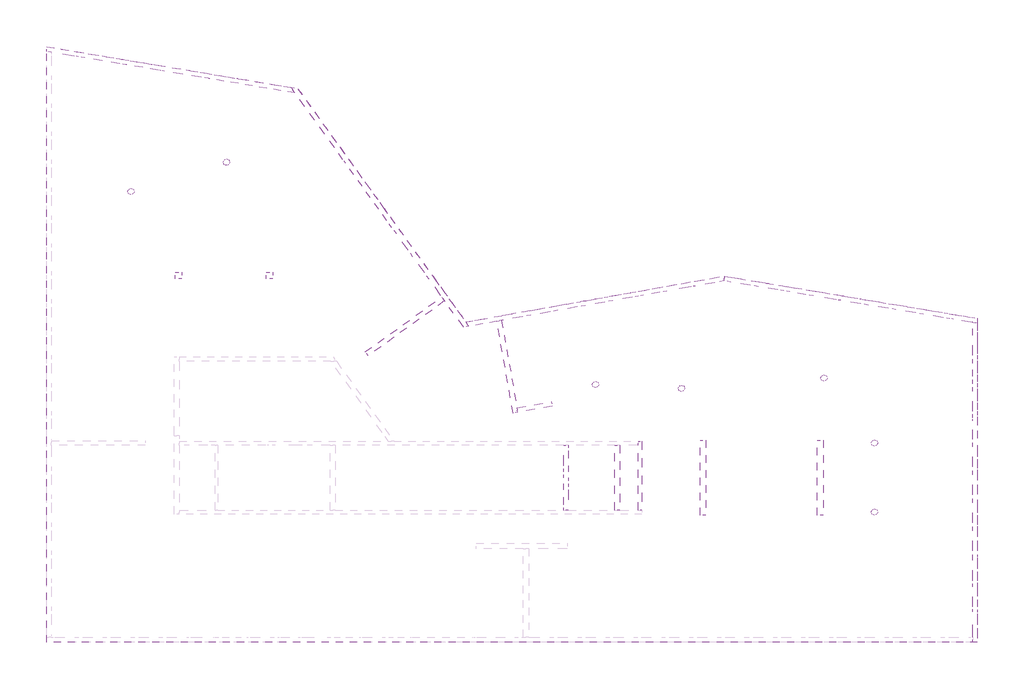
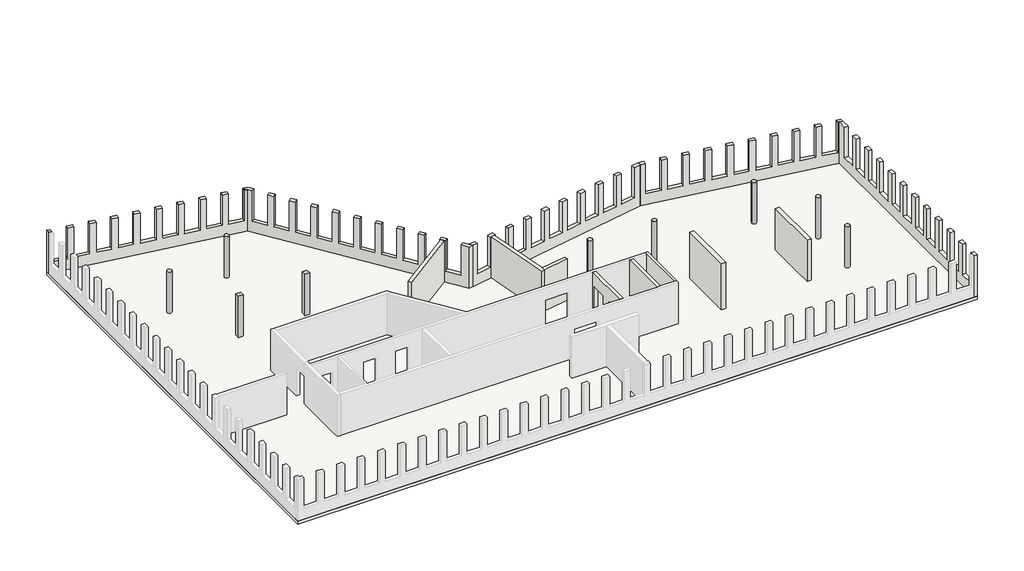
# One storey, part 2 of 2: 13 walls, 9 columns, 1 slab.
"""IFC4 building model written with IfcOpenShell, lengths in millimetres."""

from ifc_helpers import new_model, si_unit, point, frame, frame_2d, origin, place, context, project, spatial, polyline, circle_curve, trimmed, segment, composite_curve, outline, extrude, faceted_brep, element, save

model = new_model("IFC4")

# Units and contexts
model_context = context("Model", 3, world=origin())
ifc_project = project(units=[si_unit("LENGTHUNIT", "METRE", prefix="MILLI")], contexts=[model_context])

# Site, building, storey
site = spatial("IfcSite", under=ifc_project)
building = spatial("IfcBuilding", under=site)
storey = spatial("IfcBuildingStorey", under=building, Name="03_OG_OKFB_10,38", Elevation=10380.0)

# Columns
placement = place(None, origin())
element("IfcColumn", 1, ObjectType="5dki STB-Stützen rund : 5dki Stütze rund ø35cm C40/50", at=placement, inside=storey, context=model_context, shape_type="SweptSolid", body=[
    extrude(outline(composite_curve([segment(trimmed(circle_curve(frame_2d((33961.7583834, 13503.0230367)), 175.0), [point((34136.7583834, 13503.0230367))], [point((33786.7583834, 13503.0230367))], False, "CARTESIAN"), True, "CONTINUOUS"), segment(trimmed(circle_curve(frame_2d((33961.7583834, 13503.0230367)), 175.0), [point((33786.7583834, 13503.0230367))], [point((34136.7583834, 13503.0230367))], False, "CARTESIAN"), True, "CONTINUOUS")], self_intersect=False)), frame((0.0, 0.0, 13690.0), z_axis=(0.0, 0.0, 1.0), x_axis=(1.0, 0.0, 0.0)), (0.0, 0.0, 1.0), 3210.0),
])
element("IfcColumn", 2, ObjectType="5dki STB-Stützen rechteckig : 5dki Stütze recht. 35x35cm C35/45", at=placement, inside=storey, context=model_context, shape_type="SweptSolid", body=[
    extrude(outline(polyline([(7139.9999521, 19742.0124565), (7139.9999521, 19392.0124565), (6789.9999521, 19392.0124565), (6789.9999521, 19742.0124565), (7139.9999521, 19742.0124565)])), frame((0.0, 0.0, 13690.0), z_axis=(0.0, 0.0, 1.0), x_axis=(1.0, 0.0, 0.0)), (0.0, 0.0, 1.0), 3210.0),
])
element("IfcColumn", 3, ObjectType="5dki STB-Stützen rechteckig : 5dki Stütze recht. 35x35cm C35/45", at=placement, inside=storey, context=model_context, shape_type="SweptSolid", body=[
    extrude(outline(polyline([(12021.4450432, 19742.0124565), (12021.4450432, 19392.0124565), (11671.4450432, 19392.0124565), (11671.4450432, 19742.0124565), (12021.4450432, 19742.0124565)])), frame((0.0, 0.0, 13690.0), z_axis=(0.0, 0.0, 1.0), x_axis=(1.0, 0.0, 0.0)), (0.0, 0.0, 1.0), 3210.0),
])
element("IfcColumn", 4, ObjectType="5dki STB-Stützen rund : 5dki Stütze rund ø35cm C40/50", at=placement, inside=storey, context=model_context, shape_type="SweptSolid", body=[
    extrude(outline(composite_curve([segment(trimmed(circle_curve(frame_2d((41616.0718251, 14052.9332427)), 175.0), [point((41791.0718251, 14052.9332427))], [point((41441.0718251, 14052.9332427))], False, "CARTESIAN"), True, "CONTINUOUS"), segment(trimmed(circle_curve(frame_2d((41616.0718251, 14052.9332427)), 175.0), [point((41441.0718251, 14052.9332427))], [point((41791.0718251, 14052.9332427))], False, "CARTESIAN"), True, "CONTINUOUS")], self_intersect=False)), frame((0.0, 0.0, 13690.0), z_axis=(0.0, 0.0, 1.0), x_axis=(1.0, 0.0, 0.0)), (0.0, 0.0, 1.0), 3210.0),
])
element("IfcColumn", 5, ObjectType="5dki STB-Stützen rund : 5dki Stütze rund ø35cm C40/50", at=placement, inside=storey, context=model_context, shape_type="SweptSolid", body=[
    extrude(outline(composite_curve([segment(trimmed(circle_curve(frame_2d((44328.9990923, 10566.8309986)), 175.0), [point((44503.9990923, 10566.8309986))], [point((44153.9990923, 10566.8309986))], False, "CARTESIAN"), True, "CONTINUOUS"), segment(trimmed(circle_curve(frame_2d((44328.9990923, 10566.8309986)), 175.0), [point((44153.9990923, 10566.8309986))], [point((44503.9990923, 10566.8309986))], False, "CARTESIAN"), True, "CONTINUOUS")], self_intersect=False)), frame((0.0, 0.0, 13690.0), z_axis=(0.0, 0.0, 1.0), x_axis=(1.0, 0.0, 0.0)), (0.0, 0.0, 1.0), 3210.0),
])
element("IfcColumn", 6, ObjectType="5dki STB-Stützen rund : 5dki Stütze rund ø35cm C40/50", at=placement, inside=storey, context=model_context, shape_type="SweptSolid", body=[
    extrude(outline(composite_curve([segment(trimmed(circle_curve(frame_2d((44328.9990923, 6852.1619165)), 175.0), [point((44503.9990923, 6852.1619165))], [point((44153.9990923, 6852.1619165))], False, "CARTESIAN"), True, "CONTINUOUS"), segment(trimmed(circle_curve(frame_2d((44328.9990923, 6852.1619165)), 175.0), [point((44153.9990923, 6852.1619165))], [point((44503.9990923, 6852.1619165))], False, "CARTESIAN"), True, "CONTINUOUS")], self_intersect=False)), frame((0.0, 0.0, 13690.0), z_axis=(0.0, 0.0, 1.0), x_axis=(1.0, 0.0, 0.0)), (0.0, 0.0, 1.0), 3210.0),
])
element("IfcColumn", 7, ObjectType="5dki STB-Stützen rund : 5dki Stütze rund ø35cm C40/50", at=placement, inside=storey, context=model_context, shape_type="SweptSolid", body=[
    extrude(outline(composite_curve([segment(trimmed(circle_curve(frame_2d((9535.2710874, 25643.9282611)), 175.0), [point((9710.2710874, 25643.9282611))], [point((9360.2710874, 25643.9282611))], False, "CARTESIAN"), True, "CONTINUOUS"), segment(trimmed(circle_curve(frame_2d((9535.2710874, 25643.9282611)), 175.0), [point((9360.2710874, 25643.9282611))], [point((9710.2710874, 25643.9282611))], False, "CARTESIAN"), True, "CONTINUOUS")], self_intersect=False)), frame((0.0, 0.0, 13690.0), z_axis=(0.0, 0.0, 1.0), x_axis=(1.0, 0.0, 0.0)), (0.0, 0.0, 1.0), 3210.0),
])
element("IfcColumn", 8, ObjectType="5dki STB-Stützen rund : 5dki Stütze rund ø35cm C40/50", at=placement, inside=storey, context=model_context, shape_type="SweptSolid", body=[
    extrude(outline(composite_curve([segment(trimmed(circle_curve(frame_2d((4404.9034618, 24066.2757931)), 175.0), [point((4579.9034618, 24066.2757931))], [point((4229.9034618, 24066.2757931))], False, "CARTESIAN"), True, "CONTINUOUS"), segment(trimmed(circle_curve(frame_2d((4404.9034618, 24066.2757931)), 175.0), [point((4229.9034618, 24066.2757931))], [point((4579.9034618, 24066.2757931))], False, "CARTESIAN"), True, "CONTINUOUS")], self_intersect=False)), frame((0.0, 0.0, 13690.0), z_axis=(0.0, 0.0, 1.0), x_axis=(1.0, 0.0, 0.0)), (0.0, 0.0, 1.0), 3210.0),
])
element("IfcColumn", 9, ObjectType="5dki STB-Stützen rund : 5dki Stütze rund ø35cm C40/50", at=placement, inside=storey, context=model_context, shape_type="SweptSolid", body=[
    extrude(outline(composite_curve([segment(trimmed(circle_curve(frame_2d((29357.7423112, 13702.251654)), 175.0), [point((29532.7423112, 13702.251654))], [point((29182.7423112, 13702.251654))], False, "CARTESIAN"), True, "CONTINUOUS"), segment(trimmed(circle_curve(frame_2d((29357.7423112, 13702.251654)), 175.0), [point((29182.7423112, 13702.251654))], [point((29532.7423112, 13702.251654))], False, "CARTESIAN"), True, "CONTINUOUS")], self_intersect=False)), frame((0.0, 0.0, 13690.0), z_axis=(0.0, 0.0, 1.0), x_axis=(1.0, 0.0, 0.0)), (0.0, 0.0, 1.0), 3210.0),
])

# Slab
element("IfcSlab", 10, ObjectType="5dki Decke Ortbeton 25cm C30/37", at=placement, inside=storey, context=model_context, shape_type="SweptSolid", body=[
    extrude(outline(polyline([(-129.9989953, 31855.7150729), (13359.8955383, 29603.0549033), (22383.5041721, 17069.4128529), (36259.9888873, 19532.5499737), (49863.9990833, 17260.8337794), (49863.9991105, -129.9989509), (-129.9989953, -129.9990284), (-129.9989953, 31855.7150729)]), holes=[polyline([(30391.9999891, 10442.0127433), (27891.9999829, 10442.0127433), (27891.9999829, 6960.0000498), (30391.9999891, 6960.0000498), (30391.9999891, 10442.0127433)]), polyline([(31641.9999382, 10442.0127483), (30641.9999891, 10442.0127483), (30641.9999891, 6960.0000511), (31641.9999382, 6960.0000511), (31641.9999382, 10442.0127483)]), polyline([(8916.9999886, 10442.0127052), (6989.9995723, 10442.0127052), (6989.9995723, 6960.0000232), (8916.9999886, 6960.0000232), (8916.9999886, 10442.0127052)]), polyline([(24127.0004657, 8820.0328918), (16927.0004692, 8820.0328918), (16927.0004692, 7020.033352), (24127.0004657, 7020.033352), (24127.0004657, 8820.0328918)])]), frame((0.0, 0.0, 13440.0), z_axis=(0.0, 0.0, 1.0), x_axis=(1.0, 0.0, 0.0)), (0.0, 0.0, 1.0), 250.0),
])

# Walls
element("IfcWall", 11, ObjectType="5dki Lochfassade 26cm C30/37", at=placement, inside=storey, context=model_context, shape_type="Brep", body=[
    faceted_brep([(12995.7423601, 29663.864375, 13690.0), (13211.4553837, 29364.2425792, 13690.0), (22268.004401, 16784.8468851, 13690.0), (22268.004401, 16784.8468851, 16900.0), (21924.4906268, 17261.9817942, 16900.0), (21924.4906268, 17261.9817942, 14550.0), (21293.4697845, 18138.4592307, 14550.0), (21293.4697845, 18138.4592307, 16900.0), (21048.0727903, 18479.3115671, 16900.0), (21048.0727903, 18479.3115671, 14550.0), (20417.0519481, 19355.7890035, 14550.0), (20417.0519481, 19355.7890035, 16900.0), (20171.6549538, 19696.64134, 16900.0), (20171.6549538, 19696.64134, 14550.0), (19540.6341116, 20573.1187764, 14550.0), (19540.6341116, 20573.1187764, 16900.0), (19295.2371174, 20913.9711128, 16900.0), (19295.2371174, 20913.9711128, 14550.0), (18664.2162751, 21790.4485493, 14550.0), (18664.2162751, 21790.4485493, 16900.0), (18418.8192809, 22131.3008857, 16900.0), (18418.8192809, 22131.3008857, 14550.0), (17787.7984387, 23007.7783222, 14550.0), (17787.7984387, 23007.7783222, 16900.0), (17542.4014445, 23348.6306586, 16900.0), (17542.4014445, 23348.6306586, 14550.0), (16911.3806022, 24225.1080951, 14550.0), (16911.3806022, 24225.1080951, 16900.0), (16665.983608, 24565.9604315, 16900.0), (16665.983608, 24565.9604315, 14550.0), (16034.9627658, 25442.4378679, 14550.0), (16034.9627658, 25442.4378679, 16900.0), (15789.5657715, 25783.2902043, 16900.0), (15789.5657715, 25783.2902043, 14550.0), (15158.5449293, 26659.7676408, 14550.0), (15158.5449293, 26659.7676408, 16900.0), (14913.1479351, 27000.6199772, 16900.0), (14913.1479351, 27000.6199772, 14550.0), (14282.1270928, 27877.0974137, 14550.0), (14282.1270928, 27877.0974137, 16900.0), (14036.7300986, 28217.9497501, 16900.0), (14036.7300986, 28217.9497501, 14550.0), (13405.7092564, 29094.4271866, 14550.0), (13405.7092564, 29094.4271866, 16900.0), (13211.4553837, 29364.2425792, 16900.0), (13028.1664453, 29618.8278609, 16900.0), (13028.1664453, 29618.8278609, 14550.0), (12995.7423601, 29663.864375, 14550.0), (22552.0750732, 16835.2706799, 13690.0), (22383.5041721, 17069.4128529, 13690.0), (13359.8955383, 29603.0549033, 13690.0), (13359.8955383, 29603.0549033, 16900.0), (13616.7130837, 29246.3396115, 16900.0), (13616.7130837, 29246.3396115, 14550.0), (14247.7339259, 28369.8621751, 14550.0), (14247.7339259, 28369.8621751, 16900.0), (14493.1309201, 28029.0098387, 16900.0), (14493.1309201, 28029.0098387, 14550.0), (15124.1517624, 27152.5324022, 14550.0), (15124.1517624, 27152.5324022, 16900.0), (15369.5487566, 26811.6800658, 16900.0), (15369.5487566, 26811.6800658, 14550.0), (16000.5695988, 25935.2026293, 14550.0), (16000.5695988, 25935.2026293, 16900.0), (16245.966593, 25594.3502929, 16900.0), (16245.966593, 25594.3502929, 14550.0), (16876.9874353, 24717.8728564, 14550.0), (16876.9874353, 24717.8728564, 16900.0), (17122.3844295, 24377.02052, 16900.0), (17122.3844295, 24377.02052, 14550.0), (17753.4052718, 23500.5430836, 14550.0), (17753.4052718, 23500.5430836, 16900.0), (17998.802266, 23159.6907472, 16900.0), (17998.802266, 23159.6907472, 14550.0), (18629.8231082, 22283.2133107, 14550.0), (18629.8231082, 22283.2133107, 16900.0), (18875.2201024, 21942.3609743, 16900.0), (18875.2201024, 21942.3609743, 14550.0), (19506.2409447, 21065.8835378, 14550.0), (19506.2409447, 21065.8835378, 16900.0), (19751.6379389, 20725.0312014, 16900.0), (19751.6379389, 20725.0312014, 14550.0), (20382.6587811, 19848.5537649, 14550.0), (20382.6587811, 19848.5537649, 16900.0), (20628.0557754, 19507.7014285, 16900.0), (20628.0557754, 19507.7014285, 14550.0), (21259.0766176, 18631.2239921, 14550.0), (21259.0766176, 18631.2239921, 16900.0), (21504.4736118, 18290.3716557, 16900.0), (21504.4736118, 18290.3716557, 14550.0), (22135.4944541, 17413.8942192, 14550.0), (22135.4944541, 17413.8942192, 16900.0), (22383.5041721, 17069.4128529, 16900.0), (22552.0750732, 16835.2706799, 16900.0), (13034.6033862, 29657.3750221, 16900.0), (13034.6033862, 29657.3750221, 14550.0)], [[[0, 1, 2, 3, 4, 5, 6, 7, 8, 9, 10, 11, 12, 13, 14, 15, 16, 17, 18, 19, 20, 21, 22, 23, 24, 25, 26, 27, 28, 29, 30, 31, 32, 33, 34, 35, 36, 37, 38, 39, 40, 41, 42, 43, 44, 45, 46, 47]], [[48, 49, 50, 51, 52, 53, 54, 55, 56, 57, 58, 59, 60, 61, 62, 63, 64, 65, 66, 67, 68, 69, 70, 71, 72, 73, 74, 75, 76, 77, 78, 79, 80, 81, 82, 83, 84, 85, 86, 87, 88, 89, 90, 91, 92, 93]], [[2, 1, 0, 50, 49, 48]], [[3, 93, 92, 91, 4]], [[52, 51, 94, 45, 44, 43]], [[55, 40, 39, 56]], [[59, 36, 35, 60]], [[63, 32, 31, 64]], [[67, 28, 27, 68]], [[71, 24, 23, 72]], [[75, 20, 19, 76]], [[79, 16, 15, 80]], [[83, 12, 11, 84]], [[87, 8, 7, 88]], [[3, 2, 48, 93]], [[42, 53, 52, 43]], [[54, 41, 40, 55]], [[53, 42, 41, 54]], [[39, 38, 57, 56]], [[37, 36, 59, 58]], [[38, 37, 58, 57]], [[35, 34, 61, 60]], [[33, 32, 63, 62]], [[34, 33, 62, 61]], [[31, 30, 65, 64]], [[29, 28, 67, 66]], [[30, 29, 66, 65]], [[27, 26, 69, 68]], [[25, 24, 71, 70]], [[26, 25, 70, 69]], [[23, 22, 73, 72]], [[21, 20, 75, 74]], [[22, 21, 74, 73]], [[19, 18, 77, 76]], [[17, 16, 79, 78]], [[18, 17, 78, 77]], [[15, 14, 81, 80]], [[13, 12, 83, 82]], [[14, 13, 82, 81]], [[11, 10, 85, 84]], [[9, 8, 87, 86]], [[10, 9, 86, 85]], [[7, 6, 89, 88]], [[5, 4, 91, 90]], [[6, 5, 90, 89]], [[51, 50, 0, 47, 95, 94]], [[95, 46, 45, 94]], [[46, 95, 47]]]),
])
element("IfcWall", 12, ObjectType="5dki Lochfassade 26cm C30/37", at=placement, inside=storey, context=model_context, shape_type="Brep", body=[
    faceted_brep([(27318.6765704, 17681.3634281, 16900.0), (26924.8330267, 17611.4544654, 16900.0), (26924.8330267, 17611.4544654, 14550.0), (25861.4554587, 17422.7002661, 14550.0), (25861.4554587, 17422.7002661, 16900.0), (25447.9197377, 17349.2958553, 16900.0), (25447.9197377, 17349.2958553, 14550.0), (24384.5421697, 17160.541656, 14550.0), (24384.5421697, 17160.541656, 16900.0), (24300.8505369, 17145.6860228, 16900.0), (24054.698322, 17101.9929211, 16900.0), (23971.0064488, 17087.1372452, 16900.0), (23971.0064488, 17087.1372452, 14550.0), (22907.6288807, 16898.3830459, 14550.0), (22907.6288807, 16898.3830459, 16900.0), (22552.0750732, 16835.2706799, 16900.0), (22552.0750732, 16835.2706799, 13690.0), (24054.698322, 17101.9929211, 13690.0), (24300.8505369, 17145.6860228, 13690.0), (36261.33607, 19268.7248546, 13690.0), (36261.33607, 19268.7248546, 16900.0), (35766.6205834, 19180.910678, 16900.0), (35766.6205834, 19180.910678, 14550.0), (34703.2430153, 18992.1564787, 14550.0), (34703.2430153, 18992.1564787, 16900.0), (34289.7072944, 18918.7520679, 16900.0), (34289.7072944, 18918.7520679, 14550.0), (33226.3297263, 18729.9978686, 14550.0), (33226.3297263, 18729.9978686, 16900.0), (32812.7940054, 18656.5934577, 16900.0), (32812.7940054, 18656.5934577, 14550.0), (31749.4164374, 18467.8392585, 14550.0), (31749.4164374, 18467.8392585, 16900.0), (31335.8807164, 18394.4348476, 16900.0), (31335.8807164, 18394.4348476, 14550.0), (30272.5031484, 18205.6806483, 14550.0), (30272.5031484, 18205.6806483, 16900.0), (29858.9674275, 18132.2762375, 16900.0), (29858.9674275, 18132.2762375, 14550.0), (28795.5898594, 17943.5220382, 14550.0), (28795.5898594, 17943.5220382, 16900.0), (28382.0541385, 17870.1176274, 16900.0), (28382.0541385, 17870.1176274, 14550.0), (27318.6765704, 17681.3634281, 14550.0), (26879.392201, 17867.4527688, 14550.0), (26879.392201, 17867.4527688, 16900.0), (27273.2357447, 17937.3617315, 16900.0), (27273.2357447, 17937.3617315, 14550.0), (28336.6133127, 18126.1159308, 14550.0), (28336.6133127, 18126.1159308, 16900.0), (28750.1490337, 18199.5203416, 16900.0), (28750.1490337, 18199.5203416, 14550.0), (29813.5266017, 18388.2745409, 14550.0), (29813.5266017, 18388.2745409, 16900.0), (30227.0623226, 18461.6789518, 16900.0), (30227.0623226, 18461.6789518, 14550.0), (31290.4398907, 18650.433151, 14550.0), (31290.4398907, 18650.433151, 16900.0), (31703.9756116, 18723.8375619, 16900.0), (31703.9756116, 18723.8375619, 14550.0), (32767.3531797, 18912.5917612, 14550.0), (32767.3531797, 18912.5917612, 16900.0), (33180.8889006, 18985.996172, 16900.0), (33180.8889006, 18985.996172, 14550.0), (34244.2664686, 19174.7503713, 14550.0), (34244.2664686, 19174.7503713, 16900.0), (34657.8021895, 19248.1547821, 16900.0), (34657.8021895, 19248.1547821, 14550.0), (35721.1797576, 19436.9089814, 14550.0), (35721.1797576, 19436.9089814, 16900.0), (36259.9888873, 19532.5499737, 16900.0), (36259.9888873, 19532.5499737, 13690.0), (22383.5041721, 17069.4128529, 13690.0), (22383.5041721, 17069.4128529, 16900.0), (22862.188055, 17154.3813493, 16900.0), (22862.188055, 17154.3813493, 14550.0), (23925.565623, 17343.1355486, 14550.0), (23925.565623, 17343.1355486, 16900.0), (24339.1013439, 17416.5399594, 16900.0), (24339.1013439, 17416.5399594, 14550.0), (25402.478912, 17605.2941587, 14550.0), (25402.478912, 17605.2941587, 16900.0), (25816.0146329, 17678.6985695, 16900.0), (25816.0146329, 17678.6985695, 14550.0)], [[[0, 1, 2, 3, 4, 5, 6, 7, 8, 9, 10, 11, 12, 13, 14, 15, 16, 17, 18, 19, 20, 21, 22, 23, 24, 25, 26, 27, 28, 29, 30, 31, 32, 33, 34, 35, 36, 37, 38, 39, 40, 41, 42, 43]], [[44, 45, 46, 47, 48, 49, 50, 51, 52, 53, 54, 55, 56, 57, 58, 59, 60, 61, 62, 63, 64, 65, 66, 67, 68, 69, 70, 71, 72, 73, 74, 75, 76, 77, 78, 79, 80, 81, 82, 83]], [[19, 18, 17, 16, 72, 71]], [[74, 73, 15, 14]], [[50, 49, 41, 40]], [[37, 36, 54, 53]], [[58, 57, 33, 32]], [[29, 28, 62, 61]], [[21, 20, 70, 69]], [[25, 24, 66, 65]], [[78, 77, 11, 10, 9, 8]], [[82, 81, 5, 4]], [[46, 45, 1, 0]], [[16, 15, 73, 72]], [[20, 19, 71, 70]], [[14, 13, 75, 74]], [[12, 11, 77, 76]], [[13, 12, 76, 75]], [[49, 48, 42, 41]], [[47, 46, 0, 43]], [[48, 47, 43, 42]], [[40, 39, 51, 50]], [[38, 37, 53, 52]], [[39, 38, 52, 51]], [[57, 56, 34, 33]], [[55, 54, 36, 35]], [[56, 55, 35, 34]], [[32, 31, 59, 58]], [[30, 29, 61, 60]], [[31, 30, 60, 59]], [[65, 64, 26, 25]], [[63, 62, 28, 27]], [[64, 63, 27, 26]], [[69, 68, 22, 21]], [[67, 66, 24, 23]], [[68, 67, 23, 22]], [[8, 7, 79, 78]], [[6, 5, 81, 80]], [[7, 6, 80, 79]], [[4, 3, 83, 82]], [[2, 1, 45, 44]], [[3, 2, 44, 83]]]),
])
element("IfcWall", 13, ObjectType="5dki Lochfassade 26cm C30/37", at=placement, inside=storey, context=model_context, shape_type="Brep", body=[
    faceted_brep([(49863.9990837, 16997.2336245, 16900.0), (49603.9990837, 17040.6506907, 16900.0), (49507.8677901, 17056.7035319, 16900.0), (49507.8677901, 17056.7035319, 14550.0), (48442.6180365, 17234.5882205, 14550.0), (48442.6180365, 17234.5882205, 16900.0), (48028.3542434, 17303.7655993, 16900.0), (48028.3542434, 17303.7655993, 14550.0), (46963.1044898, 17481.6502878, 14550.0), (46963.1044898, 17481.6502878, 16900.0), (46548.8406967, 17550.8276667, 16900.0), (46548.8406967, 17550.8276667, 14550.0), (45483.5909431, 17728.7123552, 14550.0), (45483.5909431, 17728.7123552, 16900.0), (45069.32715, 17797.8897341, 16900.0), (45069.32715, 17797.8897341, 14550.0), (44004.0773964, 17975.7744226, 14550.0), (44004.0773964, 17975.7744226, 16900.0), (43589.8136033, 18044.9518015, 16900.0), (43589.8136033, 18044.9518015, 14550.0), (42524.5638497, 18222.83649, 14550.0), (42524.5638497, 18222.83649, 16900.0), (42110.3000566, 18292.0138689, 16900.0), (42110.3000566, 18292.0138689, 14550.0), (41045.050303, 18469.8985574, 14550.0), (41045.050303, 18469.8985574, 16900.0), (40630.7865099, 18539.0759362, 16900.0), (40630.7865099, 18539.0759362, 14550.0), (39565.5367563, 18716.9606248, 14550.0), (39565.5367563, 18716.9606248, 16900.0), (39151.2729632, 18786.1380036, 16900.0), (39151.2729632, 18786.1380036, 14550.0), (38086.0232096, 18964.0226921, 14550.0), (38086.0232096, 18964.0226921, 16900.0), (37671.7594165, 19033.200071, 16900.0), (37671.7594165, 19033.200071, 14550.0), (36606.5096629, 19211.0847595, 14550.0), (36606.5096629, 19211.0847595, 16900.0), (36261.33607, 19268.7248546, 16900.0), (36261.33607, 19268.7248546, 13690.0), (49603.9990837, 17040.6506907, 13690.0), (49863.9990837, 16997.2336245, 13690.0), (49550.6918818, 17313.1525467, 14550.0), (49550.6918818, 17313.1525467, 16900.0), (49863.9990833, 17260.8337794, 16900.0), (49863.9990833, 17260.8337794, 13690.0), (36259.9888873, 19532.5499737, 13690.0), (36259.9888873, 19532.5499737, 16900.0), (36649.3337546, 19467.5337743, 16900.0), (36649.3337546, 19467.5337743, 14550.0), (37714.5835082, 19289.6490858, 14550.0), (37714.5835082, 19289.6490858, 16900.0), (38128.8473013, 19220.4717069, 16900.0), (38128.8473013, 19220.4717069, 14550.0), (39194.0970549, 19042.5870184, 14550.0), (39194.0970549, 19042.5870184, 16900.0), (39608.360848, 18973.4096395, 16900.0), (39608.360848, 18973.4096395, 14550.0), (40673.6106016, 18795.524951, 14550.0), (40673.6106016, 18795.524951, 16900.0), (41087.8743947, 18726.3475721, 16900.0), (41087.8743947, 18726.3475721, 14550.0), (42153.1241483, 18548.4628836, 14550.0), (42153.1241483, 18548.4628836, 16900.0), (42567.3879414, 18479.2855048, 16900.0), (42567.3879414, 18479.2855048, 14550.0), (43632.637695, 18301.4008162, 14550.0), (43632.637695, 18301.4008162, 16900.0), (44046.9014881, 18232.2234374, 16900.0), (44046.9014881, 18232.2234374, 14550.0), (45112.1512417, 18054.3387489, 14550.0), (45112.1512417, 18054.3387489, 16900.0), (45526.4150348, 17985.16137, 16900.0), (45526.4150348, 17985.16137, 14550.0), (46591.6647884, 17807.2766815, 14550.0), (46591.6647884, 17807.2766815, 16900.0), (47005.9285815, 17738.0993026, 16900.0), (47005.9285815, 17738.0993026, 14550.0), (48071.1783351, 17560.2146141, 14550.0), (48071.1783351, 17560.2146141, 16900.0), (48485.4421282, 17491.0372352, 16900.0), (48485.4421282, 17491.0372352, 14550.0)], [[[0, 1, 2, 3, 4, 5, 6, 7, 8, 9, 10, 11, 12, 13, 14, 15, 16, 17, 18, 19, 20, 21, 22, 23, 24, 25, 26, 27, 28, 29, 30, 31, 32, 33, 34, 35, 36, 37, 38, 39, 40, 41]], [[42, 43, 44, 45, 46, 47, 48, 49, 50, 51, 52, 53, 54, 55, 56, 57, 58, 59, 60, 61, 62, 63, 64, 65, 66, 67, 68, 69, 70, 71, 72, 73, 74, 75, 76, 77, 78, 79, 80, 81]], [[41, 40, 39, 46, 45]], [[48, 47, 38, 37]], [[52, 51, 34, 33]], [[56, 55, 30, 29]], [[60, 59, 26, 25]], [[64, 63, 22, 21]], [[68, 67, 18, 17]], [[72, 71, 14, 13]], [[76, 75, 10, 9]], [[80, 79, 6, 5]], [[44, 43, 2, 1, 0]], [[39, 38, 47, 46]], [[0, 41, 45, 44]], [[37, 36, 49, 48]], [[35, 34, 51, 50]], [[36, 35, 50, 49]], [[33, 32, 53, 52]], [[31, 30, 55, 54]], [[32, 31, 54, 53]], [[29, 28, 57, 56]], [[27, 26, 59, 58]], [[28, 27, 58, 57]], [[25, 24, 61, 60]], [[23, 22, 63, 62]], [[24, 23, 62, 61]], [[21, 20, 65, 64]], [[19, 18, 67, 66]], [[20, 19, 66, 65]], [[17, 16, 69, 68]], [[15, 14, 71, 70]], [[16, 15, 70, 69]], [[13, 12, 73, 72]], [[11, 10, 75, 74]], [[12, 11, 74, 73]], [[9, 8, 77, 76]], [[7, 6, 79, 78]], [[8, 7, 78, 77]], [[5, 4, 81, 80]], [[3, 2, 43, 42]], [[4, 3, 42, 81]]]),
])
element("IfcWall", 14, ObjectType="5dki Lochfassade 26cm C30/37", at=placement, inside=storey, context=model_context, shape_type="Brep", body=[
    faceted_brep([(49603.9991105, -129.9989514, 16900.0), (49603.9991101, 130.0010486, 16900.0), (49603.9991099, 277.0124979, 16900.0), (49603.9991099, 277.0124979, 14550.0), (49603.9991082, 1357.0124979, 14550.0), (49603.9991082, 1357.0124979, 16900.0), (49603.9991075, 1777.0124979, 16900.0), (49603.9991075, 1777.0124979, 14550.0), (49603.9991058, 2857.0124979, 14550.0), (49603.9991058, 2857.0124979, 16900.0), (49603.9991052, 3277.0124979, 16900.0), (49603.9991052, 3277.0124979, 14550.0), (49603.9991035, 4357.0124979, 14550.0), (49603.9991035, 4357.0124979, 16900.0), (49603.9991028, 4777.0124979, 16900.0), (49603.9991028, 4777.0124979, 14550.0), (49603.9991011, 5857.0124979, 14550.0), (49603.9991011, 5857.0124979, 16900.0), (49603.9991005, 6277.0124979, 16900.0), (49603.9991005, 6277.0124979, 14550.0), (49603.9990988, 7357.0124979, 14550.0), (49603.9990988, 7357.0124979, 16900.0), (49603.9990981, 7777.0124979, 16900.0), (49603.9990981, 7777.0124979, 14550.0), (49603.9990964, 8857.0124979, 14550.0), (49603.9990964, 8857.0124979, 16900.0), (49603.9990958, 9277.0124979, 16900.0), (49603.9990958, 9277.0124979, 14550.0), (49603.9990941, 10357.0124979, 14550.0), (49603.9990941, 10357.0124979, 16900.0), (49603.9990934, 10777.0124979, 16900.0), (49603.9990934, 10777.0124979, 14550.0), (49603.9990918, 11857.0124979, 14550.0), (49603.9990918, 11857.0124979, 16900.0), (49603.9990911, 12277.0124979, 16900.0), (49603.9990911, 12277.0124979, 14550.0), (49603.9990894, 13357.0124979, 14550.0), (49603.9990894, 13357.0124979, 16900.0), (49603.9990888, 13777.0124979, 16900.0), (49603.9990888, 13777.0124979, 14550.0), (49603.9990871, 14857.0124979, 14550.0), (49603.9990871, 14857.0124979, 16900.0), (49603.9990864, 15277.0124979, 16900.0), (49603.9990864, 15277.0124979, 14550.0), (49603.9990847, 16357.0124979, 14550.0), (49603.9990847, 16357.0124979, 16900.0), (49603.9990837, 17040.6506907, 16900.0), (49603.9990837, 17040.6506907, 13690.0), (49603.9991101, 130.0010486, 13690.0), (49603.9991105, -129.9989514, 13690.0), (49863.9991099, 277.0124983, 14550.0), (49863.9991099, 277.0124983, 16900.0), (49863.9991105, -129.9989509, 16900.0), (49863.9991105, -129.9989509, 13690.0), (49863.9990837, 16997.2336245, 13690.0), (49863.9990837, 16997.2336245, 16900.0), (49863.9990847, 16357.0124983, 16900.0), (49863.9990847, 16357.0124983, 14550.0), (49863.9990864, 15277.0124983, 14550.0), (49863.9990864, 15277.0124983, 16900.0), (49863.9990871, 14857.0124983, 16900.0), (49863.9990871, 14857.0124983, 14550.0), (49863.9990888, 13777.0124983, 14550.0), (49863.9990888, 13777.0124983, 16900.0), (49863.9990894, 13357.0124983, 16900.0), (49863.9990894, 13357.0124983, 14550.0), (49863.9990911, 12277.0124983, 14550.0), (49863.9990911, 12277.0124983, 16900.0), (49863.9990918, 11857.0124983, 16900.0), (49863.9990918, 11857.0124983, 14550.0), (49863.9990934, 10777.0124983, 14550.0), (49863.9990934, 10777.0124983, 16900.0), (49863.9990941, 10357.0124983, 16900.0), (49863.9990941, 10357.0124983, 14550.0), (49863.9990958, 9277.0124983, 14550.0), (49863.9990958, 9277.0124983, 16900.0), (49863.9990964, 8857.0124983, 16900.0), (49863.9990964, 8857.0124983, 14550.0), (49863.9990981, 7777.0124983, 14550.0), (49863.9990981, 7777.0124983, 16900.0), (49863.9990988, 7357.0124983, 16900.0), (49863.9990988, 7357.0124983, 14550.0), (49863.9991005, 6277.0124983, 14550.0), (49863.9991005, 6277.0124983, 16900.0), (49863.9991011, 5857.0124983, 16900.0), (49863.9991011, 5857.0124983, 14550.0), (49863.9991028, 4777.0124983, 14550.0), (49863.9991028, 4777.0124983, 16900.0), (49863.9991035, 4357.0124983, 16900.0), (49863.9991035, 4357.0124983, 14550.0), (49863.9991052, 3277.0124983, 14550.0), (49863.9991052, 3277.0124983, 16900.0), (49863.9991058, 2857.0124983, 16900.0), (49863.9991058, 2857.0124983, 14550.0), (49863.9991075, 1777.0124983, 14550.0), (49863.9991075, 1777.0124983, 16900.0), (49863.9991082, 1357.0124983, 16900.0), (49863.9991082, 1357.0124983, 14550.0)], [[[0, 1, 2, 3, 4, 5, 6, 7, 8, 9, 10, 11, 12, 13, 14, 15, 16, 17, 18, 19, 20, 21, 22, 23, 24, 25, 26, 27, 28, 29, 30, 31, 32, 33, 34, 35, 36, 37, 38, 39, 40, 41, 42, 43, 44, 45, 46, 47, 48, 49]], [[50, 51, 52, 53, 54, 55, 56, 57, 58, 59, 60, 61, 62, 63, 64, 65, 66, 67, 68, 69, 70, 71, 72, 73, 74, 75, 76, 77, 78, 79, 80, 81, 82, 83, 84, 85, 86, 87, 88, 89, 90, 91, 92, 93, 94, 95, 96, 97]], [[49, 48, 47, 54, 53]], [[55, 46, 45, 56]], [[42, 41, 60, 59]], [[38, 37, 64, 63]], [[34, 33, 68, 67]], [[30, 29, 72, 71]], [[26, 25, 76, 75]], [[22, 21, 80, 79]], [[18, 17, 84, 83]], [[14, 13, 88, 87]], [[10, 9, 92, 91]], [[96, 95, 6, 5]], [[52, 51, 2, 1, 0]], [[47, 46, 55, 54]], [[0, 49, 53, 52]], [[58, 43, 42, 59]], [[44, 57, 56, 45]], [[43, 58, 57, 44]], [[63, 62, 39, 38]], [[61, 60, 41, 40]], [[62, 61, 40, 39]], [[67, 66, 35, 34]], [[65, 64, 37, 36]], [[66, 65, 36, 35]], [[71, 70, 31, 30]], [[69, 68, 33, 32]], [[70, 69, 32, 31]], [[75, 74, 27, 26]], [[73, 72, 29, 28]], [[74, 73, 28, 27]], [[79, 78, 23, 22]], [[77, 76, 25, 24]], [[78, 77, 24, 23]], [[83, 82, 19, 18]], [[81, 80, 21, 20]], [[82, 81, 20, 19]], [[87, 86, 15, 14]], [[85, 84, 17, 16]], [[86, 85, 16, 15]], [[91, 90, 11, 10]], [[89, 88, 13, 12]], [[90, 89, 12, 11]], [[95, 94, 7, 6]], [[93, 92, 9, 8]], [[94, 93, 8, 7]], [[5, 4, 97, 96]], [[3, 2, 51, 50]], [[4, 3, 50, 97]]]),
])
element("IfcWall", 15, ObjectType="5dki STB-Wand Kern 25cm C30/37", at=placement, inside=storey, context=model_context, shape_type="SweptSolid", body=[
    extrude(outline(polyline([(30641.9999891, 10442.0127483), (30641.9999891, 6960.0000501), (30391.9999891, 6960.0000498), (30391.9999891, 10442.0127479), (30641.9999891, 10442.0127483)])), frame((0.0, 0.0, 13690.0), z_axis=(0.0, 0.0, 1.0), x_axis=(1.0, 0.0, 0.0)), (0.0, 0.0, 1.0), 3210.0),
])
element("IfcWall", 16, ObjectType="5dki STB-Wand Kern 25cm C30/37", at=placement, inside=storey, context=model_context, shape_type="SweptSolid", body=[
    extrude(outline(polyline([(3482.0126944, -3210.0), (-2.1e-06, -3210.0), (-2.1e-06, 0.0), (279.9681323, 0.0), (279.9681323, -2260.0), (1414.9681323, -2260.0), (1414.9681323, 0.0), (2067.1995869, 0.0), (2067.1995869, -2260.0), (3202.1995869, -2260.0), (3202.1995869, 0.0), (3482.0126944, 0.0), (3482.0126944, -3210.0)])), frame((27641.9999829, 10442.0127408, 13690.0), z_axis=(1.0, 1.6300916066412081e-09, 0.0), x_axis=(1.6300916066412081e-09, -1.0, 0.0)), (0.0, 0.0, 1.0), 250.0),
])
element("IfcWall", 17, ObjectType="5dki STB-Wand Kern 20cm C35/45", at=placement, inside=storey, context=model_context, shape_type="Brep", body=[
    faceted_brep([(31641.9999912, 10662.0127502, 13690.0), (31641.9999881, 10442.0127502, 13690.0), (31641.9999382, 6960.0000514, 13690.0), (31641.9999382, 6960.0000514, 16900.0), (31641.9999881, 10442.0127502, 16900.0), (31641.9999912, 10662.0127502, 16900.0), (31841.9999912, 10662.0127505, 13690.0), (31841.9999912, 10662.0127505, 16900.0), (31841.9999382, 6960.0000516, 16900.0), (31841.9999382, 6960.0000516, 13690.0)], [[[0, 1, 2, 3, 4, 5]], [[6, 7, 8, 9]], [[2, 1, 0, 6, 9]], [[5, 4, 3, 8, 7]], [[0, 5, 7, 6]], [[3, 2, 9, 8]]]),
])
element("IfcWall", 18, ObjectType="5dki Lochfassade 26cm C30/37", at=placement, inside=storey, context=model_context, shape_type="Brep", body=[
    faceted_brep([(8967.5024476, 30072.9348316, 14550.0), (8967.5024476, 30072.9348316, 16900.0), (8553.2386546, 30142.1122105, 16900.0), (8553.2386546, 30142.1122105, 14550.0), (7487.988901, 30319.9968993, 14550.0), (7487.988901, 30319.9968993, 16900.0), (7073.7251079, 30389.1742783, 16900.0), (7073.7251079, 30389.1742783, 14550.0), (6008.4753544, 30567.058967, 14550.0), (6008.4753544, 30567.058967, 16900.0), (5594.2115613, 30636.236346, 16900.0), (5594.2115613, 30636.236346, 14550.0), (4528.9618077, 30814.1210348, 14550.0), (4528.9618077, 30814.1210348, 16900.0), (4114.6980147, 30883.2984137, 16900.0), (4114.6980147, 30883.2984137, 14550.0), (3049.4482611, 31061.1831025, 14550.0), (3049.4482611, 31061.1831025, 16900.0), (2635.184468, 31130.3604815, 16900.0), (2635.184468, 31130.3604815, 14550.0), (1569.9347144, 31308.2451702, 14550.0), (1569.9347144, 31308.2451702, 16900.0), (1155.6709214, 31377.4225492, 16900.0), (1155.6709214, 31377.4225492, 14550.0), (90.4211678, 31555.307238, 14550.0), (90.4211678, 31555.307238, 16900.0), (-129.9989953, 31592.114918, 16900.0), (-129.9989953, 31592.114918, 13690.0), (130.0010047, 31548.6978518, 13690.0), (13211.4553837, 29364.2425792, 13690.0), (13211.4553837, 29364.2425792, 16900.0), (12991.7792945, 29400.9260074, 16900.0), (12991.7792945, 29400.9260074, 14550.0), (11926.5295409, 29578.8106961, 14550.0), (11926.5295409, 29578.8106961, 16900.0), (11512.2657479, 29647.9880751, 16900.0), (11512.2657479, 29647.9880751, 14550.0), (10447.0159943, 29825.8727639, 14550.0), (10447.0159943, 29825.8727639, 16900.0), (10032.7522012, 29895.0501428, 16900.0), (10032.7522012, 29895.0501428, 14550.0), (8596.0627463, 30398.5612253, 16900.0), (9010.3265394, 30329.3838463, 16900.0), (9010.3265394, 30329.3838463, 14550.0), (10075.576293, 30151.4991576, 14550.0), (10075.576293, 30151.4991576, 16900.0), (10489.840086, 30082.3217786, 16900.0), (10489.840086, 30082.3217786, 14550.0), (11555.0898396, 29904.4370898, 14550.0), (11555.0898396, 29904.4370898, 16900.0), (11969.3536327, 29835.2597109, 16900.0), (11969.3536327, 29835.2597109, 14550.0), (12995.7423601, 29663.864375, 14550.0), (12995.7423601, 29663.864375, 13690.0), (-129.9989953, 31855.7150729, 13690.0), (-129.9989953, 31855.7150729, 16900.0), (133.2452595, 31811.7562527, 16900.0), (133.2452595, 31811.7562527, 14550.0), (1198.4950131, 31633.8715639, 14550.0), (1198.4950131, 31633.8715639, 16900.0), (1612.7588062, 31564.694185, 16900.0), (1612.7588062, 31564.694185, 14550.0), (2678.0085598, 31386.8094962, 14550.0), (2678.0085598, 31386.8094962, 16900.0), (3092.2723528, 31317.6321172, 16900.0), (3092.2723528, 31317.6321172, 14550.0), (4157.5221064, 31139.7474285, 14550.0), (4157.5221064, 31139.7474285, 16900.0), (4571.7858995, 31070.5700495, 16900.0), (4571.7858995, 31070.5700495, 14550.0), (5637.035653, 30892.6853608, 14550.0), (5637.035653, 30892.6853608, 16900.0), (6051.2994461, 30823.5079818, 16900.0), (6051.2994461, 30823.5079818, 14550.0), (7116.5491997, 30645.623293, 14550.0), (7116.5491997, 30645.623293, 16900.0), (7530.8129927, 30576.4459141, 16900.0), (7530.8129927, 30576.4459141, 14550.0), (8596.0627463, 30398.5612253, 14550.0), (13028.1664453, 29618.8278609, 16900.0), (13028.1664453, 29618.8278609, 14550.0)], [[[0, 1, 2, 3, 4, 5, 6, 7, 8, 9, 10, 11, 12, 13, 14, 15, 16, 17, 18, 19, 20, 21, 22, 23, 24, 25, 26, 27, 28, 29, 30, 31, 32, 33, 34, 35, 36, 37, 38, 39, 40]], [[41, 42, 43, 44, 45, 46, 47, 48, 49, 50, 51, 52, 53, 54, 55, 56, 57, 58, 59, 60, 61, 62, 63, 64, 65, 66, 67, 68, 69, 70, 71, 72, 73, 74, 75, 76, 77, 78]], [[29, 28, 27, 54, 53]], [[49, 35, 34, 50]], [[22, 21, 60, 59]], [[18, 17, 64, 63]], [[14, 13, 68, 67]], [[10, 9, 72, 71]], [[6, 5, 76, 75]], [[39, 38, 46, 45]], [[2, 1, 42, 41]], [[31, 30, 79]], [[55, 26, 25, 56]], [[37, 47, 46, 38]], [[48, 36, 35, 49]], [[47, 37, 36, 48]], [[58, 23, 22, 59]], [[24, 57, 56, 25]], [[23, 58, 57, 24]], [[63, 62, 19, 18]], [[61, 60, 21, 20]], [[62, 61, 20, 19]], [[67, 66, 15, 14]], [[65, 64, 17, 16]], [[66, 65, 16, 15]], [[71, 70, 11, 10]], [[69, 68, 13, 12]], [[70, 69, 12, 11]], [[75, 74, 7, 6]], [[73, 72, 9, 8]], [[74, 73, 8, 7]], [[41, 78, 3, 2]], [[77, 76, 5, 4]], [[78, 77, 4, 3]], [[45, 44, 40, 39]], [[43, 42, 1, 0]], [[44, 43, 0, 40]], [[30, 29, 53, 52, 80, 79]], [[33, 51, 50, 34]], [[80, 32, 31, 79]], [[51, 33, 32, 80, 52]], [[27, 26, 55, 54]]]),
])
element("IfcWall", 19, ObjectType="5dki STB-Wand 25cm C30/37", at=placement, inside=storey, context=model_context, shape_type="SweptSolid", body=[
    extrude(outline(polyline([(16994.6178661, 15452.6713643), (21084.845921, 18397.4352698), (21230.9155592, 18194.5469734), (17140.6875043, 15249.783068), (16994.6178661, 15452.6713643)])), frame((0.0, 0.0, 13690.0), z_axis=(0.0, 0.0, 1.0), x_axis=(1.0, 0.0, 0.0)), (0.0, 0.0, 1.0), 3210.0),
])
element("IfcWall", 20, ObjectType="5dki STB-Wand 25cm C30/37", at=placement, inside=storey, context=model_context, shape_type="Brep", body=[
    faceted_brep([(24054.698322, 17101.9929211, 13690.0), (24930.952116, 12165.4742089, 13690.0), (24930.952116, 12165.4742089, 16900.0), (24054.698322, 17101.9929211, 16900.0), (24300.8505369, 17145.6860228, 13690.0), (24300.8505369, 17145.6860228, 16900.0), (25133.4112296, 12455.3195251, 16900.0), (25177.1043309, 12209.1673103, 16900.0), (25177.1043309, 12209.1673103, 13690.0), (25133.4112296, 12455.3195251, 13690.0)], [[[0, 1, 2, 3]], [[4, 5, 6, 7, 8, 9]], [[1, 0, 4, 9, 8]], [[3, 2, 7, 6, 5]], [[0, 3, 5, 4]], [[2, 1, 8, 7]]]),
])
element("IfcWall", 21, ObjectType="5dki STB-Wand 25cm C30/37", at=placement, inside=storey, context=model_context, shape_type="SweptSolid", body=[
    extrude(outline(polyline([(27026.4023238, 12537.4258416), (25177.1043309, 12209.1673103), (25133.4112296, 12455.3195251), (26982.7092225, 12783.5780565), (27026.4023238, 12537.4258416)])), frame((0.0, 0.0, 13690.0), z_axis=(0.0, 0.0, 1.0), x_axis=(1.0, 0.0, 0.0)), (0.0, 0.0, 1.0), 3210.0),
])
element("IfcWall", 22, ObjectType="5dki STB-Wand 30cm C30/37", at=placement, inside=storey, context=model_context, shape_type="SweptSolid", body=[
    extrude(outline(polyline([(34969.9990839, 6680.0000532), (34969.9990776, 10702.0125181), (35269.9990776, 10702.0125186), (35269.9990839, 6680.0000537), (34969.9990839, 6680.0000532)])), frame((0.0, 0.0, 13690.0), z_axis=(0.0, 0.0, 1.0), x_axis=(1.0, 0.0, 0.0)), (0.0, 0.0, 1.0), 3610.0),
])
element("IfcWall", 23, ObjectType="5dki STB-Wand 30cm C30/37", at=placement, inside=storey, context=model_context, shape_type="SweptSolid", body=[
    extrude(outline(polyline([(41269.9990703, 6680.000074), (41269.9990703, 10722.0122605), (41569.9990703, 10722.0122605), (41569.9990703, 6680.000074), (41269.9990703, 6680.000074)])), frame((0.0, 0.0, 13690.0), z_axis=(0.0, 0.0, 1.0), x_axis=(1.0, 0.0, 0.0)), (0.0, 0.0, 1.0), 3210.0),
])

save(model, "model.ifc")

# Revit data of these elements
# Type "5dki STB-Stützen rund : 5dki Stütze rund ø35cm C40/50"
#   cpiFitMatchKey = "5D-KI-STB-OB-ST-RUN"
#   cpiComponentType = "Column"
#   5d Materialgüte = "C40/50"
#   Radius = 0.175 m
#   Durchmesser = 0.350 m
#   5dki Bewehrung Stab kg pro m3 = 0
#   5dki Sichtbeton SB3/SB4 [instance default] = no
#   Structural Material = 5d Beton - Stahlbeton
#   Assembly Code = ""
# Type "5dki STB-Stützen rechteckig : 5dki Stütze recht. 35x35cm C35/45"
#   cpiFitMatchKey = "5D-KI-STB-OB-ST-REC"
#   cpiComponentType = "Column"
#   5d Materialgüte = "C35/45"
#   Tiefe = 0.350 m
#   Breite = 0.350 m
#   5dki Bewehrung Stab kg pro m3 = 0
#   5dki Sichtbeton SB3/SB4 [instance default] = no
#   Structural Material = 5d Beton - Stahlbeton
#   Assembly Code = ""
# Type "5dki Decke Ortbeton 25cm C30/37"
#   cpiComponentType = "Slab"
#   cpiFitMatchKey = "5D-KI-STB-OB-DE"
#   5d Materialgüte = "C30/37"
#   Function = 0
#   5dki WU = no
#   Layers, outside or top first: 0.250 m "5d Beton - Stahlbeton" (function 1)
# Type "5dki Lochfassade 26cm C30/37"
#   Type Comments = ""
#   Description = ""
#   cpiComponentType = "Wall"
#   cpiFitMatchKey = "5D-KI-STB-OB-W-LF"
#   5d Materialgüte = "C35/45"
#   Filter Tragend / Nichttragend = yes
#   5dki WU = no
#   Layers, outside or top first: 0.260 m "5d Beton - Stahlbeton" (function 1)
# Type "5dki STB-Wand Kern 25cm C30/37"
#   Type Comments = ""
#   Description = ""
#   cpiComponentType = "Wall"
#   cpiFitMatchKey = "5D-KI-STB-OB-W-K"
#   5d Materialgüte = "C30/37"
#   Filter Tragend / Nichttragend = yes
#   5dki WU = no
#   Layers, outside or top first: 0.250 m "5d Beton - Stahlbeton" (function 1)
# Type "5dki STB-Wand Kern 20cm C35/45"
#   Type Comments = ""
#   Description = ""
#   cpiComponentType = "Wall"
#   cpiFitMatchKey = "5D-KI-STB-OB-W-K"
#   5d Materialgüte = "C35/45"
#   Filter Tragend / Nichttragend = yes
#   5dki WU = no
#   Layers, outside or top first: 0.200 m "5d Beton - Stahlbeton" (function 1)
# Type "5dki STB-Wand 25cm C30/37"
#   Type Comments = ""
#   Description = ""
#   cpiComponentType = "Wall"
#   cpiFitMatchKey = "5D-KI-STB-OB-W"
#   5d Materialgüte = "C30/37"
#   Filter Tragend / Nichttragend = yes
#   5dki WU = no
#   Layers, outside or top first: 0.250 m "5d Beton - Stahlbeton" (function 1)
# Type "5dki STB-Wand 30cm C30/37"
#   Type Comments = ""
#   Description = ""
#   cpiComponentType = "Wall"
#   cpiFitMatchKey = "5D-KI-STB-OB-W"
#   5d Materialgüte = "C30/37"
#   Filter Tragend / Nichttragend = yes
#   5dki WU = no
#   Layers, outside or top first: 0.300 m "5d Beton - Stahlbeton" (function 1)
# Elements 1, 9 (IfcColumn, "5dki STB-Stützen rund : 5dki Stütze rund ø35cm C40/50")
#   Comments = ""
#   000_080_030_Geschoß = "04_OG"
#   5dki Sichtbeton SB3/SB4 = no
#   Phase Created = Neu
#   Materials on its faces: "5d Beton - Stahlbeton"
# Element 2 (IfcColumn, "5dki STB-Stützen rechteckig : 5dki Stütze recht. 35x35cm C35/45")
#   Comments = ""
#   000_080_030_Geschoß = "04_OG"
#   5dki Sichtbeton SB3/SB4 = no
#   Phase Created = Neu
#   Materials on its faces: "5d Beton - Stahlbeton"
# Element 3 (IfcColumn, "5dki STB-Stützen rechteckig : 5dki Stütze recht. 35x35cm C35/45")
#   000_080_030_Geschoß = "04_OG"
#   5dki Sichtbeton SB3/SB4 = no
#   Phase Created = Neu
#   Materials on its faces: "5d Beton - Stahlbeton"
# Elements 4, 5, 6, 7, 8 (IfcColumn, "5dki STB-Stützen rund : 5dki Stütze rund ø35cm C40/50")
#   000_080_030_Geschoß = "04_OG"
#   5dki Sichtbeton SB3/SB4 = no
#   Phase Created = Neu
#   Materials on its faces: "5d Beton - Stahlbeton"
# Element 10 (IfcSlab, "5dki Decke Ortbeton 25cm C30/37")
#   000_080_030_Geschoß = "03_OG"
#   built-in parameter 1001955 = 2.97613 (stored number, unit not read)
#   Height Offset From Level = 0.000 m
#   built-in parameter 1001954 = 1
#   Phase Created = Neu
#   Materials on its faces: "5d Beton - Stahlbeton"
# Elements 11, 12, 13, 14, 18 (IfcWall, "5dki Lochfassade 26cm C30/37")
#   Comments = ""
#   000_080_030_Geschoß = "04_OG"
#   Top Offset = 0.000 m
#   Base Offset = 0.000 m
#   wall height = 3.210 m
#   Phase Created = Neu
#   Base Constraint = 03_OG_OKRD_13,69
#   Top Constraint = 04_OG_UKRD_16,90
#   Materials on its faces: "5d Beton - Stahlbeton"
# Elements 15, 16 (IfcWall, "5dki STB-Wand Kern 25cm C30/37")
#   Comments = ""
#   000_080_030_Geschoß = "04_OG"
#   Top Offset = 0.000 m
#   Base Offset = 0.000 m
#   wall height = 3.210 m
#   Phase Created = Neu
#   Base Constraint = 03_OG_OKRD_13,69
#   Top Constraint = 04_OG_UKRD_16,90
#   Materials on its faces: "5d Beton - Stahlbeton"
# Element 17 (IfcWall, "5dki STB-Wand Kern 20cm C35/45")
#   Comments = ""
#   000_080_030_Geschoß = "04_OG"
#   Top Offset = 0.000 m
#   Base Offset = 0.000 m
#   wall height = 3.210 m
#   Phase Created = Neu
#   Base Constraint = 03_OG_OKRD_13,69
#   Top Constraint = 04_OG_UKRD_16,90
#   Materials on its faces: "5d Beton - Stahlbeton"
# Elements 19, 20 (IfcWall, "5dki STB-Wand 25cm C30/37")
#   Comments = ""
#   000_080_030_Geschoß = "04_OG"
#   Top Offset = 0.000 m
#   Base Offset = 0.000 m
#   wall height = 3.210 m
#   Phase Created = Neu
#   Base Constraint = 03_OG_OKRD_13,69
#   Top Constraint = 04_OG_UKRD_16,90
#   Materials on its faces: "5d Beton - Stahlbeton"
# Element 21 (IfcWall, "5dki STB-Wand 25cm C30/37")
#   000_080_030_Geschoß = "04_OG"
#   Top Offset = 0.000 m
#   Base Offset = 0.000 m
#   wall height = 3.210 m
#   Phase Created = Neu
#   Base Constraint = 03_OG_OKRD_13,69
#   Top Constraint = 04_OG_UKRD_16,90
#   Materials on its faces: "5d Beton - Stahlbeton"
# Element 22 (IfcWall, "5dki STB-Wand 30cm C30/37")
#   000_080_030_Geschoß = "04_OG"
#   Top Offset = 0.400 m
#   Base Offset = 0.000 m
#   wall height = 3.610 m
#   Phase Created = Neu
#   Base Constraint = 03_OG_OKRD_13,69
#   Top Constraint = 04_OG_UKRD_16,90
#   Materials on its faces: "5d Beton - Stahlbeton"
# Element 23 (IfcWall, "5dki STB-Wand 30cm C30/37")
#   Comments = ""
#   000_080_030_Geschoß = "04_OG"
#   Top Offset = 0.000 m
#   Base Offset = 0.000 m
#   wall height = 3.210 m
#   Phase Created = Neu
#   Base Constraint = 03_OG_OKRD_13,69
#   Top Constraint = 04_OG_UKRD_16,90
#   Materials on its faces: "5d Beton - Stahlbeton"
# Materials
#   "5d Beton - Stahlbeton": class "5dki", colour RGB 200 200 200, transparency 0, Cost = 0
